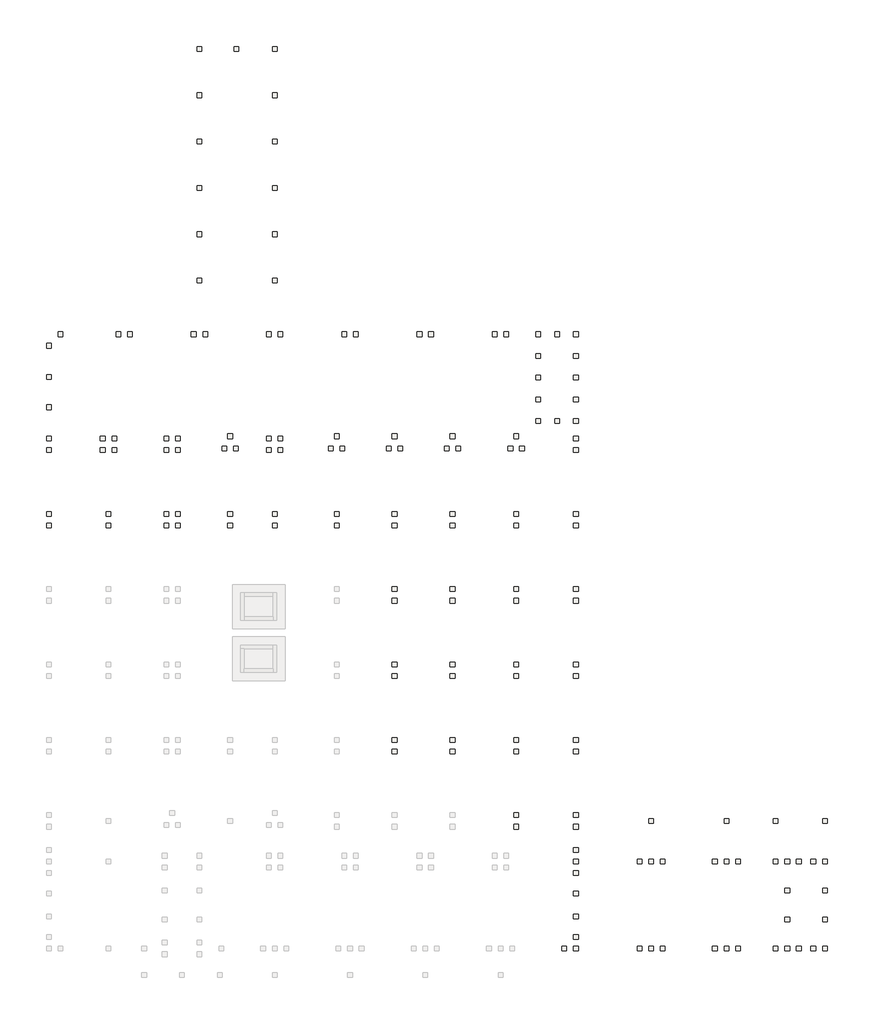
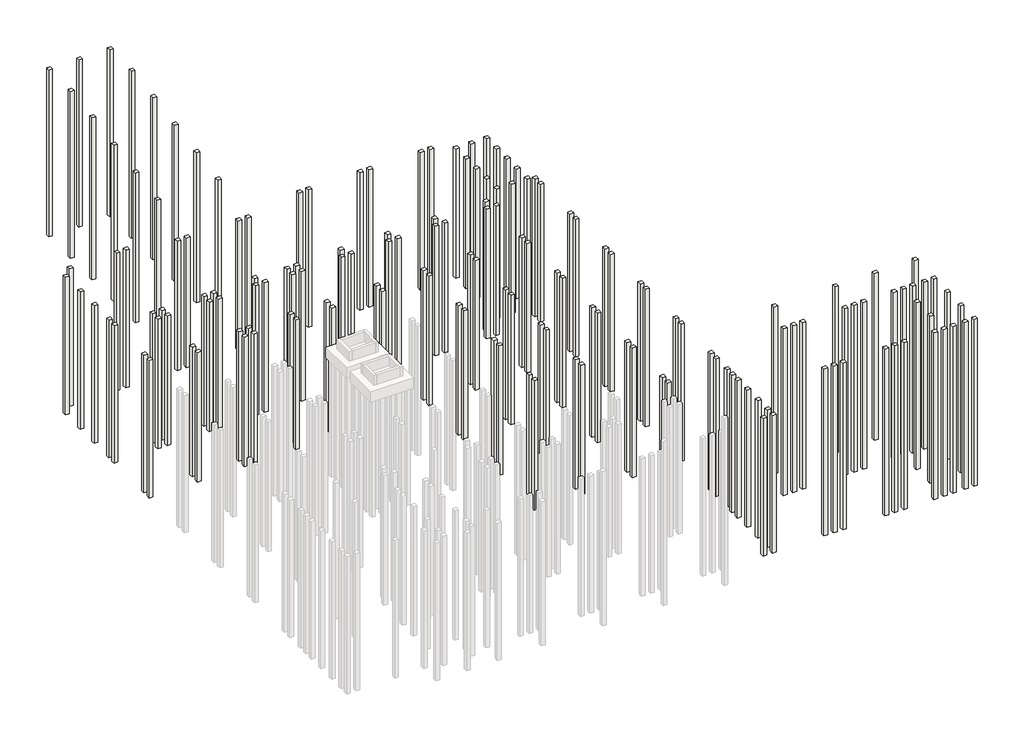
# Not in any storey, part 2 of 2: 160 footings.
"""IFC4 building model written with IfcOpenShell, lengths in millimetres."""

import ifcopenshell
import ifcopenshell.guid

model = None  # the IFC model being written
_history = None  # IfcOwnerHistory: only IFC2X3 demands one
_inside = {}  # id of a spatial element -> (the spatial element, [elements in it])
_under = {}  # id of a project, library or spatial element -> (it, [spatial elements below it])
_declared = {}  # id of a project -> (the project, [libraries it declares])
_typed = {}  # id of a type object -> (the type object, [elements of that type])
_made_of = {}  # id of a material, layer set ... -> (it, [elements and type objects made of it])


def new_model(schema):
    """Start an empty IFC model of exactly this schema.

    Asked for "IFC4X3", IfcOpenShell would pick the latest addendum, in which some entities
    have other attributes; the version numbers below select the first issue.
    IFC2X3 requires an IfcOwnerHistory on every rooted entity: one is made here for all.
    """
    global model, _history
    if schema == "IFC4X3":
        model = ifcopenshell.file(schema_version=(4, 3, 0, 0))
    else:
        model = ifcopenshell.file(schema=schema)
    _inside.clear()
    _under.clear()
    _declared.clear()
    _typed.clear()
    _made_of.clear()
    _history = None
    if model.schema == "IFC2X3":
        org = make("IfcOrganization", Name="unknown")
        user = make(
            "IfcPersonAndOrganization",
            ThePerson=make("IfcPerson", FamilyName="unknown"),
            TheOrganization=org,
        )
        app = make(
            "IfcApplication",
            ApplicationDeveloper=org,
            Version="unknown",
            ApplicationFullName="unknown",
            ApplicationIdentifier="unknown",
        )
        _history = make(
            "IfcOwnerHistory",
            OwningUser=user,
            OwningApplication=app,
            ChangeAction="ADDED",
            CreationDate=0,
        )
    return model


def make(cls, **values):
    """One entity of the class cls with the attributes given. An attribute that is None is left unset."""
    return model.create_entity(
        cls, **{name: value for name, value in values.items() if value is not None}
    )


def rooted(cls, **values):
    """An entity with a GlobalId (a new one), such as an element, a storey or a relation."""
    return make(cls, GlobalId=ifcopenshell.guid.new(), OwnerHistory=_history, **values)


def si_unit(unit_type, name, prefix=None):
    """IfcSIUnit, for example si_unit("LENGTHUNIT", "METRE", prefix="MILLI")."""
    return make("IfcSIUnit", UnitType=unit_type, Prefix=prefix, Name=name)


def assignment(units):
    """IfcUnitAssignment: the units of a project."""
    return None if units is None else make("IfcUnitAssignment", Units=units)


def point(xyz):
    """IfcCartesianPoint."""
    return None if xyz is None else make("IfcCartesianPoint", Coordinates=xyz)


def direction(xyz):
    """IfcDirection."""
    return None if xyz is None else make("IfcDirection", DirectionRatios=xyz)


def frame(location, z_axis=None, x_axis=None):
    """IfcAxis2Placement3D, a coordinate frame: its origin and axes. An axis left out is left unset."""
    return make(
        "IfcAxis2Placement3D",
        Location=point(location),
        Axis=direction(z_axis),
        RefDirection=direction(x_axis),
    )


def origin():
    """The frame at (0, 0, 0) with its axes left unset."""
    return frame((0.0, 0.0, 0.0))


def place(relative_to, where):
    """IfcLocalPlacement: puts the frame where relative to a parent placement (None: the world)."""
    return make(
        "IfcLocalPlacement", PlacementRelTo=relative_to, RelativePlacement=where
    )


def context(
    kind, dimensions, precision=None, world=None, true_north=None, identifier=None
):
    """IfcGeometricRepresentationContext, for example the 3D "Model" context."""
    return make(
        "IfcGeometricRepresentationContext",
        ContextIdentifier=identifier,
        ContextType=kind,
        CoordinateSpaceDimension=dimensions,
        Precision=precision,
        WorldCoordinateSystem=world,
        TrueNorth=true_north,
    )


def project(units=None, contexts=None):
    """IfcProject with its units and contexts."""
    return rooted(
        "IfcProject",
        Name="project",
        RepresentationContexts=contexts,
        UnitsInContext=assignment(units),
    )


def spatial(cls, under=None, at=None, **own):
    """A site, building, storey or space (cls), placed at a placement, below another one or the project."""
    s = rooted(cls, ObjectPlacement=at, **own)
    if under is not None:
        _under.setdefault(under.id(), (under, []))[1].append(s)
    return s


def polyline(points):
    """IfcPolyline through the points."""
    return make("IfcPolyline", Points=[point(p) for p in points])


def outline(outer, holes=None, kind="AREA"):
    """IfcArbitraryClosedProfileDef: a profile drawn as a closed curve; with holes, ...WithVoids."""
    if holes is None:
        return make("IfcArbitraryClosedProfileDef", ProfileType=kind, OuterCurve=outer)
    return make(
        "IfcArbitraryProfileDefWithVoids",
        ProfileType=kind,
        OuterCurve=outer,
        InnerCurves=holes,
    )


def extrude(swept, where, along, depth):
    """IfcExtrudedAreaSolid: the profile swept, set in the frame where, extruded along a direction by depth."""
    return make(
        "IfcExtrudedAreaSolid",
        SweptArea=swept,
        Position=where,
        ExtrudedDirection=direction(along),
        Depth=depth,
    )


def shape(context_of_items, identifier, shape_type, items):
    """IfcShapeRepresentation: the items that make up one representation, for example the "Body"."""
    return make(
        "IfcShapeRepresentation",
        ContextOfItems=context_of_items,
        RepresentationIdentifier=identifier,
        RepresentationType=shape_type,
        Items=items,
    )


def source(mapping_origin, context_of_items, identifier, shape_type, items):
    """IfcRepresentationMap: a shape defined once, which mapped items show again and again."""
    return make(
        "IfcRepresentationMap",
        MappingOrigin=mapping_origin,
        MappedRepresentation=shape(context_of_items, identifier, shape_type, items),
    )


def transform(
    local_origin,
    x_axis=None,
    y_axis=None,
    z_axis=None,
    scale=None,
    scale2=None,
    scale3=None,
    uniform=True,
):
    """IfcCartesianTransformationOperator3D, or its non-uniform kind. x_axis, y_axis, z_axis: its Axis1, 2, 3."""
    if uniform:
        return make(
            "IfcCartesianTransformationOperator3D",
            Axis1=direction(x_axis),
            Axis2=direction(y_axis),
            LocalOrigin=point(local_origin),
            Scale=scale,
            Axis3=direction(z_axis),
        )
    return make(
        "IfcCartesianTransformationOperator3DnonUniform",
        Axis1=direction(x_axis),
        Axis2=direction(y_axis),
        LocalOrigin=point(local_origin),
        Scale=scale,
        Axis3=direction(z_axis),
        Scale2=scale2,
        Scale3=scale3,
    )


def mapped(mapping_source, mapping_target):
    """IfcMappedItem: shows the shape of a source again, moved by a transform."""
    return make(
        "IfcMappedItem", MappingSource=mapping_source, MappingTarget=mapping_target
    )


def made_of(thing, what):
    """Note that an element or type object is made of a material, layer set ...; save() writes the relation."""
    if what is not None:
        _made_of.setdefault(what.id(), (what, []))[1].append(thing)
    return thing


def element(
    cls,
    number,
    at=None,
    inside=None,
    cuts=None,
    type_object=None,
    material=None,
    context=None,
    identifier="Body",
    shape_type=None,
    held_by="IfcProductDefinitionShape",
    body=None,
    shapes=None,
    **own,
):
    """One element of the class cls, such as IfcWall. Its Tag is "e" and its number.

    at: its placement. inside: the storey or other place that contains it. cuts: it is an
    opening in that element (IfcRelVoidsElement). A single representation is given by context,
    identifier, shape_type and body (its items); several are given by shapes. held_by: the class
    of the entity that holds the representations. save() writes the other relations.
    """
    e = rooted(cls, Tag="e%d" % number, ObjectPlacement=at, **own)
    if body is not None:
        shapes = [shape(context, identifier, shape_type, body)]
    if shapes is not None:
        e.Representation = make(held_by, Representations=shapes)
    if inside is not None:
        _inside.setdefault(inside.id(), (inside, []))[1].append(e)
    if cuts is not None:
        rooted(
            "IfcRelVoidsElement", RelatingBuildingElement=cuts, RelatedOpeningElement=e
        )
    if type_object is not None:
        _typed.setdefault(type_object.id(), (type_object, []))[1].append(e)
    return made_of(e, material)


def aggregate(whole, parts):
    """IfcRelAggregates: a whole, such as a stair, and the parts it consists of."""
    return rooted("IfcRelAggregates", RelatingObject=whole, RelatedObjects=parts)


def save(model, path):
    """Write the relations noted so far, then the file.

    IfcRelAggregates (storeys below a building ...), IfcRelContainedInSpatialStructure (elements
    in a storey), IfcRelDefinesByType, IfcRelAssociatesMaterial and IfcRelDeclares: one each for
    every whole, place, type object, material and project.
    """
    for whole, parts in _under.values():
        aggregate(whole, parts)
    for where, things in _inside.values():
        rooted(
            "IfcRelContainedInSpatialStructure",
            RelatedElements=things,
            RelatingStructure=where,
        )
    for kind, things in _typed.values():
        rooted("IfcRelDefinesByType", RelatedObjects=things, RelatingType=kind)
    for what, things in _made_of.values():
        rooted("IfcRelAssociatesMaterial", RelatedObjects=things, RelatingMaterial=what)
    for by, libraries in _declared.values():
        rooted("IfcRelDeclares", RelatingContext=by, RelatedDefinitions=libraries)
    model.write(path)


def footing_2462c6b3(model_context):
    return source(origin(), model_context, "Body", "SweptSolid", [
        extrude(outline(polyline([(200.0, -200.0), (-200.0, -200.0), (-200.0, 200.0), (200.0, 200.0), (200.0, -200.0)])), frame((0.0, 0.0, -20000.0), z_axis=(0.0, 0.0, 1.0), x_axis=(1.0, 0.0, 0.0)), (0.0, 0.0, 1.0), 14620.0),
    ])


def footing_4eaa82be(model_context):
    return source(origin(), model_context, "Body", "SweptSolid", [
        extrude(outline(polyline([(200.0, -200.0), (-200.0, -200.0), (-200.0, 200.0), (200.0, 200.0), (200.0, -200.0)])), frame((0.0, 0.0, -20000.0), z_axis=(0.0, 0.0, 1.0), x_axis=(1.0, 0.0, 0.0)), (0.0, 0.0, 1.0), 15520.0),
    ])


def footing_c87ae41e(model_context):
    return source(origin(), model_context, "Body", "SweptSolid", [
        extrude(outline(polyline([(200.0, -200.0), (-200.0, -200.0), (-200.0, 200.0), (200.0, 200.0), (200.0, -200.0)])), frame((0.0, 0.0, -20000.0), z_axis=(0.0, 0.0, 1.0), x_axis=(1.0, 0.0, 0.0)), (0.0, 0.0, 1.0), 18830.0),
    ])


def footing_0d914d5e(model_context):
    return source(origin(), model_context, "Body", "SweptSolid", [
        extrude(outline(polyline([(200.0, -200.0), (-200.0, -200.0), (-200.0, 200.0), (200.0, 200.0), (200.0, -200.0)])), frame((0.0, 0.0, -20000.0), z_axis=(0.0, 0.0, 1.0), x_axis=(1.0, 0.0, 0.0)), (0.0, 0.0, 1.0), 18850.0),
    ])


def footing_c32f4c5b(model_context):
    return source(origin(), model_context, "Body", "SweptSolid", [
        extrude(outline(polyline([(200.0, -200.0), (-200.0, -200.0), (-200.0, 200.0), (200.0, 200.0), (200.0, -200.0)])), frame((0.0, 0.0, -20000.0), z_axis=(0.0, 0.0, 1.0), x_axis=(1.0, 0.0, 0.0)), (0.0, 0.0, 1.0), 18290.0),
    ])


def footing_f6128070(model_context):
    return source(origin(), model_context, "Body", "SweptSolid", [
        extrude(outline(polyline([(200.0, -200.0), (-200.0, -200.0), (-200.0, 200.0), (200.0, 200.0), (200.0, -200.0)])), frame((0.0, 0.0, -20000.0), z_axis=(0.0, 0.0, 1.0), x_axis=(1.0, 0.0, 0.0)), (0.0, 0.0, 1.0), 17610.0),
    ])


def footing_f9187350(model_context):
    return source(origin(), model_context, "Body", "SweptSolid", [
        extrude(outline(polyline([(200.0, -200.0), (-200.0, -200.0), (-200.0, 200.0), (200.0, 200.0), (200.0, -200.0)])), frame((0.0, 0.0, -20000.0), z_axis=(0.0, 0.0, 1.0), x_axis=(1.0, 0.0, 0.0)), (0.0, 0.0, 1.0), 16925.0),
    ])


def footing_d279473c(model_context):
    return source(origin(), model_context, "Body", "SweptSolid", [
        extrude(outline(polyline([(200.0, -200.0), (-200.0, -200.0), (-200.0, 200.0), (200.0, 200.0), (200.0, -200.0)])), frame((0.0, 0.0, -20000.0), z_axis=(0.0, 0.0, 1.0), x_axis=(1.0, 0.0, 0.0)), (0.0, 0.0, 1.0), 16250.0),
    ])


model = new_model("IFC4")

# Units and contexts
model_context = context("Model", 3, world=origin())
ifc_project = project(units=[si_unit("LENGTHUNIT", "METRE", prefix="MILLI")], contexts=[model_context])

# Site, building
site = spatial("IfcSite", under=ifc_project)
building = spatial("IfcBuilding", under=site)

# Footings
placement = place(None, origin())
footing_shape = footing_2462c6b3(model_context)
element("IfcFooting", 1, at=placement, inside=building, context=model_context, shape_type="MappedRepresentation", body=[
    mapped(footing_shape, transform((11650.0, 36500.0, 0.0), x_axis=(1.0, 0.0, 0.0), y_axis=(0.0, 1.0, 0.0), z_axis=(0.0, 0.0, 1.0))),
])
element("IfcFooting", 2, at=placement, inside=building, context=model_context, shape_type="MappedRepresentation", body=[
    mapped(footing_shape, transform((11650.0, 37500.0, 0.0), x_axis=(1.0, 0.0, 0.0), y_axis=(0.0, 1.0, 0.0), z_axis=(0.0, 0.0, 1.0))),
])
element("IfcFooting", 3, at=placement, inside=building, context=model_context, shape_type="MappedRepresentation", body=[
    mapped(footing_shape, transform((22150.0, 36500.0, 0.0), x_axis=(1.0, 0.0, 0.0), y_axis=(0.0, 1.0, 0.0), z_axis=(0.0, 0.0, 1.0))),
])
element("IfcFooting", 4, at=placement, inside=building, context=model_context, shape_type="MappedRepresentation", body=[
    mapped(footing_shape, transform((22150.0, 37500.0, 0.0), x_axis=(1.0, 0.0, 0.0), y_axis=(0.0, 1.0, 0.0), z_axis=(0.0, 0.0, 1.0))),
])
element("IfcFooting", 5, at=placement, inside=building, context=model_context, shape_type="MappedRepresentation", body=[
    mapped(footing_shape, transform((26000.0, 36500.0, 0.0), x_axis=(1.0, 0.0, 0.0), y_axis=(0.0, 1.0, 0.0), z_axis=(0.0, 0.0, 1.0))),
])
element("IfcFooting", 6, at=placement, inside=building, context=model_context, shape_type="MappedRepresentation", body=[
    mapped(footing_shape, transform((26000.0, 37500.0, 0.0), x_axis=(1.0, 0.0, 0.0), y_axis=(0.0, 1.0, 0.0), z_axis=(0.0, 0.0, 1.0))),
])
element("IfcFooting", 7, at=placement, inside=building, context=model_context, shape_type="MappedRepresentation", body=[
    mapped(footing_shape, transform((46850.0, 10500.0, 0.0), x_axis=(1.0, 0.0, 0.0), y_axis=(0.0, 1.0, 0.0), z_axis=(0.0, 0.0, 1.0))),
])
element("IfcFooting", 8, at=placement, inside=building, context=model_context, shape_type="MappedRepresentation", body=[
    mapped(footing_shape, transform((46850.0, 11500.0, 0.0), x_axis=(1.0, 0.0, 0.0), y_axis=(0.0, 1.0, 0.0), z_axis=(0.0, 0.0, 1.0))),
])
element("IfcFooting", 9, at=placement, inside=building, context=model_context, shape_type="MappedRepresentation", body=[
    mapped(footing_shape, transform((17650.0, 36500.0, 0.0), x_axis=(1.0, 0.0, 0.0), y_axis=(0.0, 1.0, 0.0), z_axis=(0.0, 0.0, 1.0))),
])
element("IfcFooting", 10, at=placement, inside=building, context=model_context, shape_type="MappedRepresentation", body=[
    mapped(footing_shape, transform((17650.0, 37500.0, 0.0), x_axis=(1.0, 0.0, 0.0), y_axis=(0.0, 1.0, 0.0), z_axis=(0.0, 0.0, 1.0))),
])
element("IfcFooting", 11, at=placement, inside=building, context=model_context, shape_type="MappedRepresentation", body=[
    mapped(footing_shape, transform((16650.0, 36500.0, 0.0), x_axis=(1.0, 0.0, 0.0), y_axis=(0.0, 1.0, 0.0), z_axis=(0.0, 0.0, 1.0))),
])
element("IfcFooting", 12, at=placement, inside=building, context=model_context, shape_type="MappedRepresentation", body=[
    mapped(footing_shape, transform((16650.0, 37500.0, 0.0), x_axis=(1.0, 0.0, 0.0), y_axis=(0.0, 1.0, 0.0), z_axis=(0.0, 0.0, 1.0))),
])
element("IfcFooting", 13, at=placement, inside=building, context=model_context, shape_type="MappedRepresentation", body=[
    mapped(footing_shape, transform((48755.0, 45500.0, 0.0), x_axis=(1.0, 0.0, 0.0), y_axis=(0.0, 1.0, 0.0), z_axis=(0.0, 0.0, 1.0))),
])
element("IfcFooting", 14, at=placement, inside=building, context=model_context, shape_type="MappedRepresentation", body=[
    mapped(footing_shape, transform((52000.0, 45500.0, 0.0), x_axis=(1.0, 0.0, 0.0), y_axis=(0.0, 1.0, 0.0), z_axis=(0.0, 0.0, 1.0))),
])
element("IfcFooting", 15, at=placement, inside=building, context=model_context, shape_type="MappedRepresentation", body=[
    mapped(footing_shape, transform((52000.0, 53000.0, 0.0), x_axis=(1.0, 0.0, 0.0), y_axis=(0.0, 1.0, 0.0), z_axis=(0.0, 0.0, 1.0))),
])
element("IfcFooting", 16, at=placement, inside=building, context=model_context, shape_type="MappedRepresentation", body=[
    mapped(footing_shape, transform((48755.0, 53000.0, 0.0), x_axis=(1.0, 0.0, 0.0), y_axis=(0.0, 1.0, 0.0), z_axis=(0.0, 0.0, 1.0))),
])
element("IfcFooting", 17, at=placement, inside=building, context=model_context, shape_type="MappedRepresentation", body=[
    mapped(footing_shape, transform((50377.5, 53000.0, 0.0), x_axis=(1.0, 0.0, 0.0), y_axis=(0.0, 1.0, 0.0), z_axis=(0.0, 0.0, 1.0))),
])
element("IfcFooting", 18, at=placement, inside=building, context=model_context, shape_type="MappedRepresentation", body=[
    mapped(footing_shape, transform((50377.5, 45500.0, 0.0), x_axis=(1.0, 0.0, 0.0), y_axis=(0.0, 1.0, 0.0), z_axis=(0.0, 0.0, 1.0))),
])
element("IfcFooting", 19, at=placement, inside=building, context=model_context, shape_type="MappedRepresentation", body=[
    mapped(footing_shape, transform((48755.0, 47375.0, 0.0), x_axis=(1.0, 0.0, 0.0), y_axis=(0.0, 1.0, 0.0), z_axis=(0.0, 0.0, 1.0))),
])
element("IfcFooting", 20, at=placement, inside=building, context=model_context, shape_type="MappedRepresentation", body=[
    mapped(footing_shape, transform((48755.0, 49250.0, 0.0), x_axis=(1.0, 0.0, 0.0), y_axis=(0.0, 1.0, 0.0), z_axis=(0.0, 0.0, 1.0))),
])
element("IfcFooting", 21, at=placement, inside=building, context=model_context, shape_type="MappedRepresentation", body=[
    mapped(footing_shape, transform((48755.0, 51125.0, 0.0), x_axis=(1.0, 0.0, 0.0), y_axis=(0.0, 1.0, 0.0), z_axis=(0.0, 0.0, 1.0))),
])
element("IfcFooting", 22, at=placement, inside=building, context=model_context, shape_type="MappedRepresentation", body=[
    mapped(footing_shape, transform((52000.0, 47375.0, 0.0), x_axis=(1.0, 0.0, 0.0), y_axis=(0.0, 1.0, 0.0), z_axis=(0.0, 0.0, 1.0))),
])
element("IfcFooting", 23, at=placement, inside=building, context=model_context, shape_type="MappedRepresentation", body=[
    mapped(footing_shape, transform((52000.0, 49250.0, 0.0), x_axis=(1.0, 0.0, 0.0), y_axis=(0.0, 1.0, 0.0), z_axis=(0.0, 0.0, 1.0))),
])
element("IfcFooting", 24, at=placement, inside=building, context=model_context, shape_type="MappedRepresentation", body=[
    mapped(footing_shape, transform((52000.0, 51125.0, 0.0), x_axis=(1.0, 0.0, 0.0), y_axis=(0.0, 1.0, 0.0), z_axis=(0.0, 0.0, 1.0))),
])
element("IfcFooting", 25, at=placement, inside=building, context=model_context, shape_type="MappedRepresentation", body=[
    mapped(footing_shape, transform((36350.0, 17000.0, 0.0), x_axis=(1.0, 0.0, 0.0), y_axis=(0.0, 1.0, 0.0), z_axis=(0.0, 0.0, 1.0))),
])
element("IfcFooting", 26, at=placement, inside=building, context=model_context, shape_type="MappedRepresentation", body=[
    mapped(footing_shape, transform((36350.0, 18000.0, 0.0), x_axis=(1.0, 0.0, 0.0), y_axis=(0.0, 1.0, 0.0), z_axis=(0.0, 0.0, 1.0))),
])
element("IfcFooting", 27, at=placement, inside=building, context=model_context, shape_type="MappedRepresentation", body=[
    mapped(footing_shape, transform((41350.0, 17000.0, 0.0), x_axis=(1.0, 0.0, 0.0), y_axis=(0.0, 1.0, 0.0), z_axis=(0.0, 0.0, 1.0))),
])
element("IfcFooting", 28, at=placement, inside=building, context=model_context, shape_type="MappedRepresentation", body=[
    mapped(footing_shape, transform((41350.0, 18000.0, 0.0), x_axis=(1.0, 0.0, 0.0), y_axis=(0.0, 1.0, 0.0), z_axis=(0.0, 0.0, 1.0))),
])
element("IfcFooting", 29, at=placement, inside=building, context=model_context, shape_type="MappedRepresentation", body=[
    mapped(footing_shape, transform((46850.0, 17000.0, 0.0), x_axis=(1.0, 0.0, 0.0), y_axis=(0.0, 1.0, 0.0), z_axis=(0.0, 0.0, 1.0))),
])
element("IfcFooting", 30, at=placement, inside=building, context=model_context, shape_type="MappedRepresentation", body=[
    mapped(footing_shape, transform((46850.0, 18000.0, 0.0), x_axis=(1.0, 0.0, 0.0), y_axis=(0.0, 1.0, 0.0), z_axis=(0.0, 0.0, 1.0))),
])
element("IfcFooting", 31, at=placement, inside=building, context=model_context, shape_type="MappedRepresentation", body=[
    mapped(footing_shape, transform((46850.0, 23500.0, 0.0), x_axis=(1.0, 0.0, 0.0), y_axis=(0.0, 1.0, 0.0), z_axis=(0.0, 0.0, 1.0))),
])
element("IfcFooting", 32, at=placement, inside=building, context=model_context, shape_type="MappedRepresentation", body=[
    mapped(footing_shape, transform((46850.0, 24500.0, 0.0), x_axis=(1.0, 0.0, 0.0), y_axis=(0.0, 1.0, 0.0), z_axis=(0.0, 0.0, 1.0))),
])
element("IfcFooting", 33, at=placement, inside=building, context=model_context, shape_type="MappedRepresentation", body=[
    mapped(footing_shape, transform((41350.0, 23500.0, 0.0), x_axis=(1.0, 0.0, 0.0), y_axis=(0.0, 1.0, 0.0), z_axis=(0.0, 0.0, 1.0))),
])
element("IfcFooting", 34, at=placement, inside=building, context=model_context, shape_type="MappedRepresentation", body=[
    mapped(footing_shape, transform((41350.0, 24500.0, 0.0), x_axis=(1.0, 0.0, 0.0), y_axis=(0.0, 1.0, 0.0), z_axis=(0.0, 0.0, 1.0))),
])
element("IfcFooting", 35, at=placement, inside=building, context=model_context, shape_type="MappedRepresentation", body=[
    mapped(footing_shape, transform((36350.0, 23500.0, 0.0), x_axis=(1.0, 0.0, 0.0), y_axis=(0.0, 1.0, 0.0), z_axis=(0.0, 0.0, 1.0))),
])
element("IfcFooting", 36, at=placement, inside=building, context=model_context, shape_type="MappedRepresentation", body=[
    mapped(footing_shape, transform((36350.0, 24500.0, 0.0), x_axis=(1.0, 0.0, 0.0), y_axis=(0.0, 1.0, 0.0), z_axis=(0.0, 0.0, 1.0))),
])
element("IfcFooting", 37, at=placement, inside=building, context=model_context, shape_type="MappedRepresentation", body=[
    mapped(footing_shape, transform((36350.0, 30000.0, 0.0), x_axis=(1.0, 0.0, 0.0), y_axis=(0.0, 1.0, 0.0), z_axis=(0.0, 0.0, 1.0))),
])
element("IfcFooting", 38, at=placement, inside=building, context=model_context, shape_type="MappedRepresentation", body=[
    mapped(footing_shape, transform((36350.0, 31000.0, 0.0), x_axis=(1.0, 0.0, 0.0), y_axis=(0.0, 1.0, 0.0), z_axis=(0.0, 0.0, 1.0))),
])
element("IfcFooting", 39, at=placement, inside=building, context=model_context, shape_type="MappedRepresentation", body=[
    mapped(footing_shape, transform((41350.0, 30000.0, 0.0), x_axis=(1.0, 0.0, 0.0), y_axis=(0.0, 1.0, 0.0), z_axis=(0.0, 0.0, 1.0))),
])
element("IfcFooting", 40, at=placement, inside=building, context=model_context, shape_type="MappedRepresentation", body=[
    mapped(footing_shape, transform((41350.0, 31000.0, 0.0), x_axis=(1.0, 0.0, 0.0), y_axis=(0.0, 1.0, 0.0), z_axis=(0.0, 0.0, 1.0))),
])
element("IfcFooting", 41, at=placement, inside=building, context=model_context, shape_type="MappedRepresentation", body=[
    mapped(footing_shape, transform((46850.0, 30000.0, 0.0), x_axis=(1.0, 0.0, 0.0), y_axis=(0.0, 1.0, 0.0), z_axis=(0.0, 0.0, 1.0))),
])
element("IfcFooting", 42, at=placement, inside=building, context=model_context, shape_type="MappedRepresentation", body=[
    mapped(footing_shape, transform((46850.0, 31000.0, 0.0), x_axis=(1.0, 0.0, 0.0), y_axis=(0.0, 1.0, 0.0), z_axis=(0.0, 0.0, 1.0))),
])
element("IfcFooting", 43, at=placement, inside=building, context=model_context, shape_type="MappedRepresentation", body=[
    mapped(footing_shape, transform((46850.0, 36500.0, 0.0), x_axis=(1.0, 0.0, 0.0), y_axis=(0.0, 1.0, 0.0), z_axis=(0.0, 0.0, 1.0))),
])
element("IfcFooting", 44, at=placement, inside=building, context=model_context, shape_type="MappedRepresentation", body=[
    mapped(footing_shape, transform((46850.0, 37500.0, 0.0), x_axis=(1.0, 0.0, 0.0), y_axis=(0.0, 1.0, 0.0), z_axis=(0.0, 0.0, 1.0))),
])
element("IfcFooting", 45, at=placement, inside=building, context=model_context, shape_type="MappedRepresentation", body=[
    mapped(footing_shape, transform((41350.0, 36500.0, 0.0), x_axis=(1.0, 0.0, 0.0), y_axis=(0.0, 1.0, 0.0), z_axis=(0.0, 0.0, 1.0))),
])
element("IfcFooting", 46, at=placement, inside=building, context=model_context, shape_type="MappedRepresentation", body=[
    mapped(footing_shape, transform((41350.0, 37500.0, 0.0), x_axis=(1.0, 0.0, 0.0), y_axis=(0.0, 1.0, 0.0), z_axis=(0.0, 0.0, 1.0))),
])
element("IfcFooting", 47, at=placement, inside=building, context=model_context, shape_type="MappedRepresentation", body=[
    mapped(footing_shape, transform((36350.0, 36500.0, 0.0), x_axis=(1.0, 0.0, 0.0), y_axis=(0.0, 1.0, 0.0), z_axis=(0.0, 0.0, 1.0))),
])
element("IfcFooting", 48, at=placement, inside=building, context=model_context, shape_type="MappedRepresentation", body=[
    mapped(footing_shape, transform((36350.0, 37500.0, 0.0), x_axis=(1.0, 0.0, 0.0), y_axis=(0.0, 1.0, 0.0), z_axis=(0.0, 0.0, 1.0))),
])
element("IfcFooting", 49, at=placement, inside=building, context=model_context, shape_type="MappedRepresentation", body=[
    mapped(footing_shape, transform((31350.0, 36500.0, 0.0), x_axis=(1.0, 0.0, 0.0), y_axis=(0.0, 1.0, 0.0), z_axis=(0.0, 0.0, 1.0))),
])
element("IfcFooting", 50, at=placement, inside=building, context=model_context, shape_type="MappedRepresentation", body=[
    mapped(footing_shape, transform((31350.0, 37500.0, 0.0), x_axis=(1.0, 0.0, 0.0), y_axis=(0.0, 1.0, 0.0), z_axis=(0.0, 0.0, 1.0))),
])
element("IfcFooting", 51, at=placement, inside=building, context=model_context, shape_type="MappedRepresentation", body=[
    mapped(footing_shape, transform((12150.0, 43000.0, 0.0), x_axis=(1.0, 0.0, 0.0), y_axis=(0.0, 1.0, 0.0), z_axis=(0.0, 0.0, 1.0))),
])
element("IfcFooting", 52, at=placement, inside=building, context=model_context, shape_type="MappedRepresentation", body=[
    mapped(footing_shape, transform((12150.0, 44000.0, 0.0), x_axis=(1.0, 0.0, 0.0), y_axis=(0.0, 1.0, 0.0), z_axis=(0.0, 0.0, 1.0))),
])
element("IfcFooting", 53, at=placement, inside=building, context=model_context, shape_type="MappedRepresentation", body=[
    mapped(footing_shape, transform((11150.0, 43000.0, 0.0), x_axis=(1.0, 0.0, 0.0), y_axis=(0.0, 1.0, 0.0), z_axis=(0.0, 0.0, 1.0))),
])
element("IfcFooting", 54, at=placement, inside=building, context=model_context, shape_type="MappedRepresentation", body=[
    mapped(footing_shape, transform((11150.0, 44000.0, 0.0), x_axis=(1.0, 0.0, 0.0), y_axis=(0.0, 1.0, 0.0), z_axis=(0.0, 0.0, 1.0))),
])
element("IfcFooting", 55, at=placement, inside=building, context=model_context, shape_type="MappedRepresentation", body=[
    mapped(footing_shape, transform((17650.0, 43000.0, 0.0), x_axis=(1.0, 0.0, 0.0), y_axis=(0.0, 1.0, 0.0), z_axis=(0.0, 0.0, 1.0))),
])
element("IfcFooting", 56, at=placement, inside=building, context=model_context, shape_type="MappedRepresentation", body=[
    mapped(footing_shape, transform((17650.0, 44000.0, 0.0), x_axis=(1.0, 0.0, 0.0), y_axis=(0.0, 1.0, 0.0), z_axis=(0.0, 0.0, 1.0))),
])
element("IfcFooting", 57, at=placement, inside=building, context=model_context, shape_type="MappedRepresentation", body=[
    mapped(footing_shape, transform((16650.0, 43000.0, 0.0), x_axis=(1.0, 0.0, 0.0), y_axis=(0.0, 1.0, 0.0), z_axis=(0.0, 0.0, 1.0))),
])
element("IfcFooting", 58, at=placement, inside=building, context=model_context, shape_type="MappedRepresentation", body=[
    mapped(footing_shape, transform((16650.0, 44000.0, 0.0), x_axis=(1.0, 0.0, 0.0), y_axis=(0.0, 1.0, 0.0), z_axis=(0.0, 0.0, 1.0))),
])
element("IfcFooting", 59, at=placement, inside=building, context=model_context, shape_type="MappedRepresentation", body=[
    mapped(footing_shape, transform((21650.0, 43150.0, 0.0), x_axis=(1.0, 0.0, 0.0), y_axis=(0.0, 1.0, 0.0), z_axis=(0.0, 0.0, 1.0))),
])
element("IfcFooting", 60, at=placement, inside=building, context=model_context, shape_type="MappedRepresentation", body=[
    mapped(footing_shape, transform((22650.0, 43150.0, 0.0), x_axis=(1.0, 0.0, 0.0), y_axis=(0.0, 1.0, 0.0), z_axis=(0.0, 0.0, 1.0))),
])
element("IfcFooting", 61, at=placement, inside=building, context=model_context, shape_type="MappedRepresentation", body=[
    mapped(footing_shape, transform((22150.0, 44200.0, 0.0), x_axis=(1.0, 0.0, 0.0), y_axis=(0.0, 1.0, 0.0), z_axis=(0.0, 0.0, 1.0))),
])
element("IfcFooting", 62, at=placement, inside=building, context=model_context, shape_type="MappedRepresentation", body=[
    mapped(footing_shape, transform((26500.0, 43000.0, 0.0), x_axis=(1.0, 0.0, 0.0), y_axis=(0.0, 1.0, 0.0), z_axis=(0.0, 0.0, 1.0))),
])
element("IfcFooting", 63, at=placement, inside=building, context=model_context, shape_type="MappedRepresentation", body=[
    mapped(footing_shape, transform((26500.0, 44000.0, 0.0), x_axis=(1.0, 0.0, 0.0), y_axis=(0.0, 1.0, 0.0), z_axis=(0.0, 0.0, 1.0))),
])
element("IfcFooting", 64, at=placement, inside=building, context=model_context, shape_type="MappedRepresentation", body=[
    mapped(footing_shape, transform((25500.0, 43000.0, 0.0), x_axis=(1.0, 0.0, 0.0), y_axis=(0.0, 1.0, 0.0), z_axis=(0.0, 0.0, 1.0))),
])
element("IfcFooting", 65, at=placement, inside=building, context=model_context, shape_type="MappedRepresentation", body=[
    mapped(footing_shape, transform((25500.0, 44000.0, 0.0), x_axis=(1.0, 0.0, 0.0), y_axis=(0.0, 1.0, 0.0), z_axis=(0.0, 0.0, 1.0))),
])
element("IfcFooting", 66, at=placement, inside=building, context=model_context, shape_type="MappedRepresentation", body=[
    mapped(footing_shape, transform((30850.0, 43150.0, 0.0), x_axis=(1.0, 0.0, 0.0), y_axis=(0.0, 1.0, 0.0), z_axis=(0.0, 0.0, 1.0))),
])
element("IfcFooting", 67, at=placement, inside=building, context=model_context, shape_type="MappedRepresentation", body=[
    mapped(footing_shape, transform((31850.0, 43150.0, 0.0), x_axis=(1.0, 0.0, 0.0), y_axis=(0.0, 1.0, 0.0), z_axis=(0.0, 0.0, 1.0))),
])
element("IfcFooting", 68, at=placement, inside=building, context=model_context, shape_type="MappedRepresentation", body=[
    mapped(footing_shape, transform((31350.0, 44200.0, 0.0), x_axis=(1.0, 0.0, 0.0), y_axis=(0.0, 1.0, 0.0), z_axis=(0.0, 0.0, 1.0))),
])
element("IfcFooting", 69, at=placement, inside=building, context=model_context, shape_type="MappedRepresentation", body=[
    mapped(footing_shape, transform((35850.0, 43150.0, 0.0), x_axis=(1.0, 0.0, 0.0), y_axis=(0.0, 1.0, 0.0), z_axis=(0.0, 0.0, 1.0))),
])
element("IfcFooting", 70, at=placement, inside=building, context=model_context, shape_type="MappedRepresentation", body=[
    mapped(footing_shape, transform((36850.0, 43150.0, 0.0), x_axis=(1.0, 0.0, 0.0), y_axis=(0.0, 1.0, 0.0), z_axis=(0.0, 0.0, 1.0))),
])
element("IfcFooting", 71, at=placement, inside=building, context=model_context, shape_type="MappedRepresentation", body=[
    mapped(footing_shape, transform((36350.0, 44200.0, 0.0), x_axis=(1.0, 0.0, 0.0), y_axis=(0.0, 1.0, 0.0), z_axis=(0.0, 0.0, 1.0))),
])
element("IfcFooting", 72, at=placement, inside=building, context=model_context, shape_type="MappedRepresentation", body=[
    mapped(footing_shape, transform((40850.0, 43150.0, 0.0), x_axis=(1.0, 0.0, 0.0), y_axis=(0.0, 1.0, 0.0), z_axis=(0.0, 0.0, 1.0))),
])
element("IfcFooting", 73, at=placement, inside=building, context=model_context, shape_type="MappedRepresentation", body=[
    mapped(footing_shape, transform((41850.0, 43150.0, 0.0), x_axis=(1.0, 0.0, 0.0), y_axis=(0.0, 1.0, 0.0), z_axis=(0.0, 0.0, 1.0))),
])
element("IfcFooting", 74, at=placement, inside=building, context=model_context, shape_type="MappedRepresentation", body=[
    mapped(footing_shape, transform((41350.0, 44200.0, 0.0), x_axis=(1.0, 0.0, 0.0), y_axis=(0.0, 1.0, 0.0), z_axis=(0.0, 0.0, 1.0))),
])
element("IfcFooting", 75, at=placement, inside=building, context=model_context, shape_type="MappedRepresentation", body=[
    mapped(footing_shape, transform((46350.0, 43150.0, 0.0), x_axis=(1.0, 0.0, 0.0), y_axis=(0.0, 1.0, 0.0), z_axis=(0.0, 0.0, 1.0))),
])
element("IfcFooting", 76, at=placement, inside=building, context=model_context, shape_type="MappedRepresentation", body=[
    mapped(footing_shape, transform((47350.0, 43150.0, 0.0), x_axis=(1.0, 0.0, 0.0), y_axis=(0.0, 1.0, 0.0), z_axis=(0.0, 0.0, 1.0))),
])
element("IfcFooting", 77, at=placement, inside=building, context=model_context, shape_type="MappedRepresentation", body=[
    mapped(footing_shape, transform((46850.0, 44200.0, 0.0), x_axis=(1.0, 0.0, 0.0), y_axis=(0.0, 1.0, 0.0), z_axis=(0.0, 0.0, 1.0))),
])
element("IfcFooting", 78, at=placement, inside=building, context=model_context, shape_type="MappedRepresentation", body=[
    mapped(footing_shape, transform((25500.0, 53000.0, 0.0), x_axis=(1.0, 0.0, 0.0), y_axis=(0.0, 1.0, 0.0), z_axis=(0.0, 0.0, 1.0))),
])
element("IfcFooting", 79, at=placement, inside=building, context=model_context, shape_type="MappedRepresentation", body=[
    mapped(footing_shape, transform((26500.0, 53000.0, 0.0), x_axis=(1.0, 0.0, 0.0), y_axis=(0.0, 1.0, 0.0), z_axis=(0.0, 0.0, 1.0))),
])
element("IfcFooting", 80, at=placement, inside=building, context=model_context, shape_type="MappedRepresentation", body=[
    mapped(footing_shape, transform((19000.0, 53000.0, 0.0), x_axis=(1.0, 0.0, 0.0), y_axis=(0.0, 1.0, 0.0), z_axis=(0.0, 0.0, 1.0))),
])
element("IfcFooting", 81, at=placement, inside=building, context=model_context, shape_type="MappedRepresentation", body=[
    mapped(footing_shape, transform((20000.0, 53000.0, 0.0), x_axis=(1.0, 0.0, 0.0), y_axis=(0.0, 1.0, 0.0), z_axis=(0.0, 0.0, 1.0))),
])
footing_2_shape = footing_4eaa82be(model_context)
element("IfcFooting", 82, at=placement, inside=building, context=model_context, shape_type="MappedRepresentation", body=[
    mapped(footing_2_shape, transform((7500.0, 53000.0, 0.0), x_axis=(1.0, 0.0, 0.0), y_axis=(0.0, 1.0, 0.0), z_axis=(0.0, 0.0, 1.0))),
])
element("IfcFooting", 83, at=placement, inside=building, context=model_context, shape_type="MappedRepresentation", body=[
    mapped(footing_2_shape, transform((6500.0, 52000.0, 0.0), x_axis=(1.0, 0.0, 0.0), y_axis=(0.0, 1.0, 0.0), z_axis=(0.0, 0.0, 1.0))),
])
element("IfcFooting", 84, at=placement, inside=building, context=model_context, shape_type="MappedRepresentation", body=[
    mapped(footing_2_shape, transform((6500.0, 43000.0, 0.0), x_axis=(1.0, 0.0, 0.0), y_axis=(0.0, 1.0, 0.0), z_axis=(0.0, 0.0, 1.0))),
])
element("IfcFooting", 85, at=placement, inside=building, context=model_context, shape_type="MappedRepresentation", body=[
    mapped(footing_2_shape, transform((6500.0, 44000.0, 0.0), x_axis=(1.0, 0.0, 0.0), y_axis=(0.0, 1.0, 0.0), z_axis=(0.0, 0.0, 1.0))),
])
element("IfcFooting", 86, at=placement, inside=building, context=model_context, shape_type="MappedRepresentation", body=[
    mapped(footing_2_shape, transform((6500.0, 46700.0, 0.0), x_axis=(1.0, 0.0, 0.0), y_axis=(0.0, 1.0, 0.0), z_axis=(0.0, 0.0, 1.0))),
])
element("IfcFooting", 87, at=placement, inside=building, context=model_context, shape_type="MappedRepresentation", body=[
    mapped(footing_2_shape, transform((52000.0, 43000.0, 0.0), x_axis=(1.0, 0.0, 0.0), y_axis=(0.0, 1.0, 0.0), z_axis=(0.0, 0.0, 1.0))),
])
element("IfcFooting", 88, at=placement, inside=building, context=model_context, shape_type="MappedRepresentation", body=[
    mapped(footing_2_shape, transform((52000.0, 44000.0, 0.0), x_axis=(1.0, 0.0, 0.0), y_axis=(0.0, 1.0, 0.0), z_axis=(0.0, 0.0, 1.0))),
])
element("IfcFooting", 89, at=placement, inside=building, context=model_context, shape_type="MappedRepresentation", body=[
    mapped(footing_2_shape, transform((51000.0, 0.0, 0.0), x_axis=(1.0, 0.0, 0.0), y_axis=(0.0, 1.0, 0.0), z_axis=(0.0, 0.0, 1.0))),
])
element("IfcFooting", 90, at=placement, inside=building, context=model_context, shape_type="MappedRepresentation", body=[
    mapped(footing_2_shape, transform((52000.0, 0.0, 0.0), x_axis=(1.0, 0.0, 0.0), y_axis=(0.0, 1.0, 0.0), z_axis=(0.0, 0.0, 1.0))),
])
element("IfcFooting", 91, at=placement, inside=building, context=model_context, shape_type="MappedRepresentation", body=[
    mapped(footing_2_shape, transform((52000.0, 1000.0, 0.0), x_axis=(1.0, 0.0, 0.0), y_axis=(0.0, 1.0, 0.0), z_axis=(0.0, 0.0, 1.0))),
])
element("IfcFooting", 92, at=placement, inside=building, context=model_context, shape_type="MappedRepresentation", body=[
    mapped(footing_2_shape, transform((52000.0, 2750.0, 0.0), x_axis=(1.0, 0.0, 0.0), y_axis=(0.0, 1.0, 0.0), z_axis=(0.0, 0.0, 1.0))),
])
element("IfcFooting", 93, at=placement, inside=building, context=model_context, shape_type="MappedRepresentation", body=[
    mapped(footing_2_shape, transform((52000.0, 6500.0, 0.0), x_axis=(1.0, 0.0, 0.0), y_axis=(0.0, 1.0, 0.0), z_axis=(0.0, 0.0, 1.0))),
])
element("IfcFooting", 94, at=placement, inside=building, context=model_context, shape_type="MappedRepresentation", body=[
    mapped(footing_2_shape, transform((52000.0, 7500.0, 0.0), x_axis=(1.0, 0.0, 0.0), y_axis=(0.0, 1.0, 0.0), z_axis=(0.0, 0.0, 1.0))),
])
element("IfcFooting", 95, at=placement, inside=building, context=model_context, shape_type="MappedRepresentation", body=[
    mapped(footing_2_shape, transform((52000.0, 8500.0, 0.0), x_axis=(1.0, 0.0, 0.0), y_axis=(0.0, 1.0, 0.0), z_axis=(0.0, 0.0, 1.0))),
])
element("IfcFooting", 96, at=placement, inside=building, context=model_context, shape_type="MappedRepresentation", body=[
    mapped(footing_2_shape, transform((52000.0, 4750.0, 0.0), x_axis=(1.0, 0.0, 0.0), y_axis=(0.0, 1.0, 0.0), z_axis=(0.0, 0.0, 1.0))),
])
element("IfcFooting", 97, at=placement, inside=building, context=model_context, shape_type="MappedRepresentation", body=[
    mapped(footing_2_shape, transform((52000.0, 10500.0, 0.0), x_axis=(1.0, 0.0, 0.0), y_axis=(0.0, 1.0, 0.0), z_axis=(0.0, 0.0, 1.0))),
])
element("IfcFooting", 98, at=placement, inside=building, context=model_context, shape_type="MappedRepresentation", body=[
    mapped(footing_2_shape, transform((52000.0, 11500.0, 0.0), x_axis=(1.0, 0.0, 0.0), y_axis=(0.0, 1.0, 0.0), z_axis=(0.0, 0.0, 1.0))),
])
element("IfcFooting", 99, at=placement, inside=building, context=model_context, shape_type="MappedRepresentation", body=[
    mapped(footing_2_shape, transform((6500.0, 36500.0, 0.0), x_axis=(1.0, 0.0, 0.0), y_axis=(0.0, 1.0, 0.0), z_axis=(0.0, 0.0, 1.0))),
])
element("IfcFooting", 100, at=placement, inside=building, context=model_context, shape_type="MappedRepresentation", body=[
    mapped(footing_2_shape, transform((6500.0, 37500.0, 0.0), x_axis=(1.0, 0.0, 0.0), y_axis=(0.0, 1.0, 0.0), z_axis=(0.0, 0.0, 1.0))),
])
element("IfcFooting", 101, at=placement, inside=building, context=model_context, shape_type="MappedRepresentation", body=[
    mapped(footing_2_shape, transform((52000.0, 17000.0, 0.0), x_axis=(1.0, 0.0, 0.0), y_axis=(0.0, 1.0, 0.0), z_axis=(0.0, 0.0, 1.0))),
])
element("IfcFooting", 102, at=placement, inside=building, context=model_context, shape_type="MappedRepresentation", body=[
    mapped(footing_2_shape, transform((52000.0, 18000.0, 0.0), x_axis=(1.0, 0.0, 0.0), y_axis=(0.0, 1.0, 0.0), z_axis=(0.0, 0.0, 1.0))),
])
element("IfcFooting", 103, at=placement, inside=building, context=model_context, shape_type="MappedRepresentation", body=[
    mapped(footing_2_shape, transform((52000.0, 23500.0, 0.0), x_axis=(1.0, 0.0, 0.0), y_axis=(0.0, 1.0, 0.0), z_axis=(0.0, 0.0, 1.0))),
])
element("IfcFooting", 104, at=placement, inside=building, context=model_context, shape_type="MappedRepresentation", body=[
    mapped(footing_2_shape, transform((52000.0, 24500.0, 0.0), x_axis=(1.0, 0.0, 0.0), y_axis=(0.0, 1.0, 0.0), z_axis=(0.0, 0.0, 1.0))),
])
element("IfcFooting", 105, at=placement, inside=building, context=model_context, shape_type="MappedRepresentation", body=[
    mapped(footing_2_shape, transform((52000.0, 30000.0, 0.0), x_axis=(1.0, 0.0, 0.0), y_axis=(0.0, 1.0, 0.0), z_axis=(0.0, 0.0, 1.0))),
])
element("IfcFooting", 106, at=placement, inside=building, context=model_context, shape_type="MappedRepresentation", body=[
    mapped(footing_2_shape, transform((52000.0, 31000.0, 0.0), x_axis=(1.0, 0.0, 0.0), y_axis=(0.0, 1.0, 0.0), z_axis=(0.0, 0.0, 1.0))),
])
element("IfcFooting", 107, at=placement, inside=building, context=model_context, shape_type="MappedRepresentation", body=[
    mapped(footing_2_shape, transform((52000.0, 36500.0, 0.0), x_axis=(1.0, 0.0, 0.0), y_axis=(0.0, 1.0, 0.0), z_axis=(0.0, 0.0, 1.0))),
])
element("IfcFooting", 108, at=placement, inside=building, context=model_context, shape_type="MappedRepresentation", body=[
    mapped(footing_2_shape, transform((52000.0, 37500.0, 0.0), x_axis=(1.0, 0.0, 0.0), y_axis=(0.0, 1.0, 0.0), z_axis=(0.0, 0.0, 1.0))),
])
element("IfcFooting", 109, at=placement, inside=building, context=model_context, shape_type="MappedRepresentation", body=[
    mapped(footing_2_shape, transform((46000.0, 53000.0, 0.0), x_axis=(1.0, 0.0, 0.0), y_axis=(0.0, 1.0, 0.0), z_axis=(0.0, 0.0, 1.0))),
])
element("IfcFooting", 110, at=placement, inside=building, context=model_context, shape_type="MappedRepresentation", body=[
    mapped(footing_2_shape, transform((45000.0, 53000.0, 0.0), x_axis=(1.0, 0.0, 0.0), y_axis=(0.0, 1.0, 0.0), z_axis=(0.0, 0.0, 1.0))),
])
element("IfcFooting", 111, at=placement, inside=building, context=model_context, shape_type="MappedRepresentation", body=[
    mapped(footing_2_shape, transform((39500.0, 53000.0, 0.0), x_axis=(1.0, 0.0, 0.0), y_axis=(0.0, 1.0, 0.0), z_axis=(0.0, 0.0, 1.0))),
])
element("IfcFooting", 112, at=placement, inside=building, context=model_context, shape_type="MappedRepresentation", body=[
    mapped(footing_2_shape, transform((38500.0, 53000.0, 0.0), x_axis=(1.0, 0.0, 0.0), y_axis=(0.0, 1.0, 0.0), z_axis=(0.0, 0.0, 1.0))),
])
element("IfcFooting", 113, at=placement, inside=building, context=model_context, shape_type="MappedRepresentation", body=[
    mapped(footing_2_shape, transform((33000.0, 53000.0, 0.0), x_axis=(1.0, 0.0, 0.0), y_axis=(0.0, 1.0, 0.0), z_axis=(0.0, 0.0, 1.0))),
])
element("IfcFooting", 114, at=placement, inside=building, context=model_context, shape_type="MappedRepresentation", body=[
    mapped(footing_2_shape, transform((32000.0, 53000.0, 0.0), x_axis=(1.0, 0.0, 0.0), y_axis=(0.0, 1.0, 0.0), z_axis=(0.0, 0.0, 1.0))),
])
element("IfcFooting", 115, at=placement, inside=building, context=model_context, shape_type="MappedRepresentation", body=[
    mapped(footing_2_shape, transform((6500.0, 49300.0, 0.0), x_axis=(1.0, 0.0, 0.0), y_axis=(0.0, 1.0, 0.0), z_axis=(0.0, 0.0, 1.0))),
])
element("IfcFooting", 116, at=placement, inside=building, context=model_context, shape_type="MappedRepresentation", body=[
    mapped(footing_2_shape, transform((13500.0, 53000.0, 0.0), x_axis=(1.0, 0.0, 0.0), y_axis=(0.0, 1.0, 0.0), z_axis=(0.0, 0.0, 1.0))),
])
element("IfcFooting", 117, at=placement, inside=building, context=model_context, shape_type="MappedRepresentation", body=[
    mapped(footing_2_shape, transform((12500.0, 53000.0, 0.0), x_axis=(1.0, 0.0, 0.0), y_axis=(0.0, 1.0, 0.0), z_axis=(0.0, 0.0, 1.0))),
])
footing_3_shape = footing_c87ae41e(model_context)
element("IfcFooting", 118, at=placement, inside=building, context=model_context, shape_type="MappedRepresentation", body=[
    mapped(footing_3_shape, transform((57500.0, 7500.0, 0.0), x_axis=(1.0, 0.0, 0.0), y_axis=(0.0, 1.0, 0.0), z_axis=(0.0, 0.0, 1.0))),
])
element("IfcFooting", 119, at=placement, inside=building, context=model_context, shape_type="MappedRepresentation", body=[
    mapped(footing_3_shape, transform((58500.0, 7500.0, 0.0), x_axis=(-1.0, 0.0, 0.0), y_axis=(0.0, -1.0, 0.0), z_axis=(0.0, 0.0, 1.0))),
])
element("IfcFooting", 120, at=placement, inside=building, context=model_context, shape_type="MappedRepresentation", body=[
    mapped(footing_3_shape, transform((59500.0, 7500.0, 0.0), x_axis=(-1.0, 0.0, 0.0), y_axis=(0.0, -1.0, 0.0), z_axis=(0.0, 0.0, 1.0))),
])
element("IfcFooting", 121, at=placement, inside=building, context=model_context, shape_type="MappedRepresentation", body=[
    mapped(footing_3_shape, transform((64000.0, 7500.0, 0.0), x_axis=(1.0, 0.0, 0.0), y_axis=(0.0, 1.0, 0.0), z_axis=(0.0, 0.0, 1.0))),
])
element("IfcFooting", 122, at=placement, inside=building, context=model_context, shape_type="MappedRepresentation", body=[
    mapped(footing_3_shape, transform((65000.0, 7500.0, 0.0), x_axis=(1.0, 0.0, 0.0), y_axis=(0.0, 1.0, 0.0), z_axis=(0.0, 0.0, 1.0))),
])
element("IfcFooting", 123, at=placement, inside=building, context=model_context, shape_type="MappedRepresentation", body=[
    mapped(footing_3_shape, transform((66000.0, 7500.0, 0.0), x_axis=(1.0, 0.0, 0.0), y_axis=(0.0, 1.0, 0.0), z_axis=(0.0, 0.0, 1.0))),
])
element("IfcFooting", 124, at=placement, inside=building, context=model_context, shape_type="MappedRepresentation", body=[
    mapped(footing_3_shape, transform((57500.0, 0.0, 0.0), x_axis=(1.0, 0.0, 0.0), y_axis=(0.0, 1.0, 0.0), z_axis=(0.0, 0.0, 1.0))),
])
element("IfcFooting", 125, at=placement, inside=building, context=model_context, shape_type="MappedRepresentation", body=[
    mapped(footing_3_shape, transform((58500.0, 0.0, 0.0), x_axis=(1.0, 0.0, 0.0), y_axis=(0.0, 1.0, 0.0), z_axis=(0.0, 0.0, 1.0))),
])
element("IfcFooting", 126, at=placement, inside=building, context=model_context, shape_type="MappedRepresentation", body=[
    mapped(footing_3_shape, transform((59500.0, 0.0, 0.0), x_axis=(1.0, 0.0, 0.0), y_axis=(0.0, 1.0, 0.0), z_axis=(0.0, 0.0, 1.0))),
])
element("IfcFooting", 127, at=placement, inside=building, context=model_context, shape_type="MappedRepresentation", body=[
    mapped(footing_3_shape, transform((64000.0, 0.0, 0.0), x_axis=(1.0, 0.0, 0.0), y_axis=(0.0, 1.0, 0.0), z_axis=(0.0, 0.0, 1.0))),
])
element("IfcFooting", 128, at=placement, inside=building, context=model_context, shape_type="MappedRepresentation", body=[
    mapped(footing_3_shape, transform((65000.0, 0.0, 0.0), x_axis=(1.0, 0.0, 0.0), y_axis=(0.0, 1.0, 0.0), z_axis=(0.0, 0.0, 1.0))),
])
element("IfcFooting", 129, at=placement, inside=building, context=model_context, shape_type="MappedRepresentation", body=[
    mapped(footing_3_shape, transform((66000.0, 0.0, 0.0), x_axis=(1.0, 0.0, 0.0), y_axis=(0.0, 1.0, 0.0), z_axis=(0.0, 0.0, 1.0))),
])
element("IfcFooting", 130, at=placement, inside=building, context=model_context, shape_type="MappedRepresentation", body=[
    mapped(footing_3_shape, transform((70250.0, 0.0, 0.0), x_axis=(1.0, 0.0, 0.0), y_axis=(0.0, 1.0, 0.0), z_axis=(0.0, 0.0, 1.0))),
])
element("IfcFooting", 131, at=placement, inside=building, context=model_context, shape_type="MappedRepresentation", body=[
    mapped(footing_3_shape, transform((71250.0, 0.0, 0.0), x_axis=(1.0, 0.0, 0.0), y_axis=(0.0, 1.0, 0.0), z_axis=(0.0, 0.0, 1.0))),
])
element("IfcFooting", 132, at=placement, inside=building, context=model_context, shape_type="MappedRepresentation", body=[
    mapped(footing_3_shape, transform((73500.0, 0.0, 0.0), x_axis=(1.0, 0.0, 0.0), y_axis=(0.0, 1.0, 0.0), z_axis=(0.0, 0.0, 1.0))),
])
element("IfcFooting", 133, at=placement, inside=building, context=model_context, shape_type="MappedRepresentation", body=[
    mapped(footing_3_shape, transform((70250.0, 7500.0, 0.0), x_axis=(1.0, 0.0, 0.0), y_axis=(0.0, 1.0, 0.0), z_axis=(0.0, 0.0, 1.0))),
])
element("IfcFooting", 134, at=placement, inside=building, context=model_context, shape_type="MappedRepresentation", body=[
    mapped(footing_3_shape, transform((71250.0, 7500.0, 0.0), x_axis=(1.0, 0.0, 0.0), y_axis=(0.0, 1.0, 0.0), z_axis=(0.0, 0.0, 1.0))),
])
element("IfcFooting", 135, at=placement, inside=building, context=model_context, shape_type="MappedRepresentation", body=[
    mapped(footing_3_shape, transform((73500.0, 7500.0, 0.0), x_axis=(1.0, 0.0, 0.0), y_axis=(0.0, 1.0, 0.0), z_axis=(0.0, 0.0, 1.0))),
])
element("IfcFooting", 136, at=placement, inside=building, context=model_context, shape_type="MappedRepresentation", body=[
    mapped(footing_3_shape, transform((70250.0, 5000.0, 0.0), x_axis=(1.0, 0.0, 0.0), y_axis=(0.0, 1.0, 0.0), z_axis=(0.0, 0.0, 1.0))),
])
element("IfcFooting", 137, at=placement, inside=building, context=model_context, shape_type="MappedRepresentation", body=[
    mapped(footing_3_shape, transform((70250.0, 2500.0, 0.0), x_axis=(1.0, 0.0, 0.0), y_axis=(0.0, 1.0, 0.0), z_axis=(0.0, 0.0, 1.0))),
])
element("IfcFooting", 138, at=placement, inside=building, context=model_context, shape_type="MappedRepresentation", body=[
    mapped(footing_3_shape, transform((73500.0, 5000.0, 0.0), x_axis=(1.0, 0.0, 0.0), y_axis=(0.0, 1.0, 0.0), z_axis=(0.0, 0.0, 1.0))),
])
element("IfcFooting", 139, at=placement, inside=building, context=model_context, shape_type="MappedRepresentation", body=[
    mapped(footing_3_shape, transform((73500.0, 2500.0, 0.0), x_axis=(1.0, 0.0, 0.0), y_axis=(0.0, 1.0, 0.0), z_axis=(0.0, 0.0, 1.0))),
])
element("IfcFooting", 140, at=placement, inside=building, context=model_context, shape_type="MappedRepresentation", body=[
    mapped(footing_3_shape, transform((69250.0, 0.0, 0.0), x_axis=(1.0, 0.0, 0.0), y_axis=(0.0, 1.0, 0.0), z_axis=(0.0, 0.0, 1.0))),
])
element("IfcFooting", 141, at=placement, inside=building, context=model_context, shape_type="MappedRepresentation", body=[
    mapped(footing_3_shape, transform((69250.0, 7500.0, 0.0), x_axis=(1.0, 0.0, 0.0), y_axis=(0.0, 1.0, 0.0), z_axis=(0.0, 0.0, 1.0))),
])
element("IfcFooting", 142, at=placement, inside=building, context=model_context, shape_type="MappedRepresentation", body=[
    mapped(footing_3_shape, transform((72500.0, 0.0, 0.0), x_axis=(1.0, 0.0, 0.0), y_axis=(0.0, 1.0, 0.0), z_axis=(0.0, 0.0, 1.0))),
])
element("IfcFooting", 143, at=placement, inside=building, context=model_context, shape_type="MappedRepresentation", body=[
    mapped(footing_3_shape, transform((72500.0, 7500.0, 0.0), x_axis=(1.0, 0.0, 0.0), y_axis=(0.0, 1.0, 0.0), z_axis=(0.0, 0.0, 1.0))),
])
element("IfcFooting", 144, at=placement, inside=building, context=model_context, shape_type="MappedRepresentation", body=[
    mapped(footing_3_shape, transform((58500.0, 11000.0, 0.0), x_axis=(-1.0, 0.0, 0.0), y_axis=(0.0, -1.0, 0.0), z_axis=(0.0, 0.0, 1.0))),
])
element("IfcFooting", 145, at=placement, inside=building, context=model_context, shape_type="MappedRepresentation", body=[
    mapped(footing_3_shape, transform((65000.0, 11000.0, 0.0), x_axis=(-1.0, 0.0, 0.0), y_axis=(0.0, -1.0, 0.0), z_axis=(0.0, 0.0, 1.0))),
])
element("IfcFooting", 146, at=placement, inside=building, context=model_context, shape_type="MappedRepresentation", body=[
    mapped(footing_3_shape, transform((69250.0, 11000.0, 0.0), x_axis=(-1.0, 0.0, 0.0), y_axis=(0.0, -1.0, 0.0), z_axis=(0.0, 0.0, 1.0))),
])
element("IfcFooting", 147, at=placement, inside=building, context=model_context, shape_type="MappedRepresentation", body=[
    mapped(footing_3_shape, transform((73500.0, 11000.0, 0.0), x_axis=(-1.0, 0.0, 0.0), y_axis=(0.0, -1.0, 0.0), z_axis=(0.0, 0.0, 1.0))),
])
footing_4_shape = footing_0d914d5e(model_context)
element("IfcFooting", 148, at=placement, inside=building, context=model_context, shape_type="MappedRepresentation", body=[
    mapped(footing_4_shape, transform((26000.0, 77620.0, 0.0), x_axis=(1.0, 0.0, 0.0), y_axis=(0.0, 1.0, 0.0), z_axis=(0.0, 0.0, 1.0))),
])
element("IfcFooting", 149, at=placement, inside=building, context=model_context, shape_type="MappedRepresentation", body=[
    mapped(footing_4_shape, transform((19500.0, 77620.0, 0.0), x_axis=(1.0, 0.0, 0.0), y_axis=(0.0, 1.0, 0.0), z_axis=(0.0, 0.0, 1.0))),
])
element("IfcFooting", 150, at=placement, inside=building, context=model_context, shape_type="MappedRepresentation", body=[
    mapped(footing_4_shape, transform((22700.0, 77620.0, 0.0), x_axis=(1.0, 0.0, 0.0), y_axis=(0.0, 1.0, 0.0), z_axis=(0.0, 0.0, 1.0))),
])
element("IfcFooting", 151, at=placement, inside=building, context=model_context, shape_type="MappedRepresentation", body=[
    mapped(footing_4_shape, transform((19500.0, 73620.0, 0.0), x_axis=(1.0, 0.0, 0.0), y_axis=(0.0, 1.0, 0.0), z_axis=(0.0, 0.0, 1.0))),
])
element("IfcFooting", 152, at=placement, inside=building, context=model_context, shape_type="MappedRepresentation", body=[
    mapped(footing_4_shape, transform((26000.0, 73620.0, 0.0), x_axis=(1.0, 0.0, 0.0), y_axis=(0.0, 1.0, 0.0), z_axis=(0.0, 0.0, 1.0))),
])
footing_5_shape = footing_c32f4c5b(model_context)
element("IfcFooting", 153, at=placement, inside=building, context=model_context, shape_type="MappedRepresentation", body=[
    mapped(footing_5_shape, transform((26000.0, 69620.0, 0.0), x_axis=(1.0, 0.0, 0.0), y_axis=(0.0, 1.0, 0.0), z_axis=(0.0, 0.0, 1.0))),
])
element("IfcFooting", 154, at=placement, inside=building, context=model_context, shape_type="MappedRepresentation", body=[
    mapped(footing_5_shape, transform((19500.0, 69620.0, 0.0), x_axis=(1.0, 0.0, 0.0), y_axis=(0.0, 1.0, 0.0), z_axis=(0.0, 0.0, 1.0))),
])
footing_6_shape = footing_f6128070(model_context)
element("IfcFooting", 155, at=placement, inside=building, context=model_context, shape_type="MappedRepresentation", body=[
    mapped(footing_6_shape, transform((26000.0, 65620.0, 0.0), x_axis=(1.0, 0.0, 0.0), y_axis=(0.0, 1.0, 0.0), z_axis=(0.0, 0.0, 1.0))),
])
element("IfcFooting", 156, at=placement, inside=building, context=model_context, shape_type="MappedRepresentation", body=[
    mapped(footing_6_shape, transform((19500.0, 65620.0, 0.0), x_axis=(1.0, 0.0, 0.0), y_axis=(0.0, 1.0, 0.0), z_axis=(0.0, 0.0, 1.0))),
])
footing_7_shape = footing_f9187350(model_context)
element("IfcFooting", 157, at=placement, inside=building, context=model_context, shape_type="MappedRepresentation", body=[
    mapped(footing_7_shape, transform((26000.0, 61620.0, 0.0), x_axis=(1.0, 0.0, 0.0), y_axis=(0.0, 1.0, 0.0), z_axis=(0.0, 0.0, 1.0))),
])
element("IfcFooting", 158, at=placement, inside=building, context=model_context, shape_type="MappedRepresentation", body=[
    mapped(footing_7_shape, transform((19500.0, 61620.0, 0.0), x_axis=(1.0, 0.0, 0.0), y_axis=(0.0, 1.0, 0.0), z_axis=(0.0, 0.0, 1.0))),
])
footing_8_shape = footing_d279473c(model_context)
element("IfcFooting", 159, at=placement, inside=building, context=model_context, shape_type="MappedRepresentation", body=[
    mapped(footing_8_shape, transform((26000.0, 57620.0, 0.0), x_axis=(1.0, 0.0, 0.0), y_axis=(0.0, 1.0, 0.0), z_axis=(0.0, 0.0, 1.0))),
])
element("IfcFooting", 160, at=placement, inside=building, context=model_context, shape_type="MappedRepresentation", body=[
    mapped(footing_8_shape, transform((19500.0, 57620.0, 0.0), x_axis=(1.0, 0.0, 0.0), y_axis=(0.0, 1.0, 0.0), z_axis=(0.0, 0.0, 1.0))),
])

save(model, "model.ifc")

# Revit data of these elements
# Type "NLRS_17_SFO_TLB_funderingspaal geheid beton prefab-AV-MMBPC_gen_rsf : heipaal beton prefab_gen__bxh 400x400"
#   IfcExportAs = "IfcPile"
#   Type Comments = "prefab heipaal 400x400"
#   Model = " "
#   Manufacturer = " "
#   Description = "prefab heipaal 400x400"
#   Assembly Code = "17.21"
#   Width = 400 mm
#   Slanted Angle [instance default] = 0.00°
#   NLRS_S_draagvermogen_trek [instance default] = 0.00 kN
#   NLRS_S_draagvermogen_druk [instance default] = 0.00 kN
#   NLRS_C_lengte [instance default] = 1660 mm
#   NLRS_C_hoogte = 400 mm
#   NLRS_C_breedte = 400 mm
#   Height [instance default] = 1660 mm
#   Length [instance default] = 1660 mm
#   Angle [instance default] = 0.00°
#   Slanted [instance default] = 0
#   Structural Material = NLRS_f2_beton prefab_gen_rsf
#   Keynote = ""
# Element 1 (IfcFooting, "NLRS_17_SFO_TLB_funderingspaal geheid beton prefab-AV-MMBPC_gen_rsf : heipaal beton prefab_gen__bxh 400x400")
#   IfcGUID = "10$Kfo5uPCAOPJEOo5LEto"
#   Slanted Angle = 0.00°
#   NLRS_S_draagvermogen_trek = 0.00 kN
#   NLRS_S_draagvermogen_druk = 0.00 kN
#   Angle = 0.00°
#   IsExternal = yes
#   LoadBearing = yes
#   Slanted = 0
#   Phase Created = NLRS_nieuw
#   Materials on its faces: "NLRS_f2_beton prefab_gen_rsf"
# Element 2 (IfcFooting, "NLRS_17_SFO_TLB_funderingspaal geheid beton prefab-AV-MMBPC_gen_rsf : heipaal beton prefab_gen__bxh 400x400")
#   IfcGUID = "10$Kfo5uPCAOPJEOo5LEtq"
#   Slanted Angle = 0.00°
#   NLRS_S_draagvermogen_trek = 0.00 kN
#   NLRS_S_draagvermogen_druk = 0.00 kN
#   Angle = 0.00°
#   IsExternal = yes
#   LoadBearing = yes
#   Slanted = 0
#   Phase Created = NLRS_nieuw
#   Materials on its faces: "NLRS_f2_beton prefab_gen_rsf"
# Element 3 (IfcFooting, "NLRS_17_SFO_TLB_funderingspaal geheid beton prefab-AV-MMBPC_gen_rsf : heipaal beton prefab_gen__bxh 400x400")
#   IfcGUID = "10$Kfo5uPCAOPJEOo5LEs1"
#   Slanted Angle = 0.00°
#   NLRS_S_draagvermogen_trek = 0.00 kN
#   NLRS_S_draagvermogen_druk = 0.00 kN
#   Angle = 0.00°
#   IsExternal = yes
#   LoadBearing = yes
#   Slanted = 0
#   Phase Created = NLRS_nieuw
#   Materials on its faces: "NLRS_f2_beton prefab_gen_rsf"
